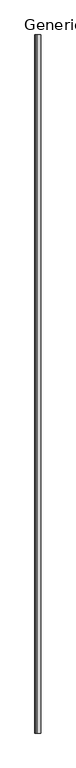
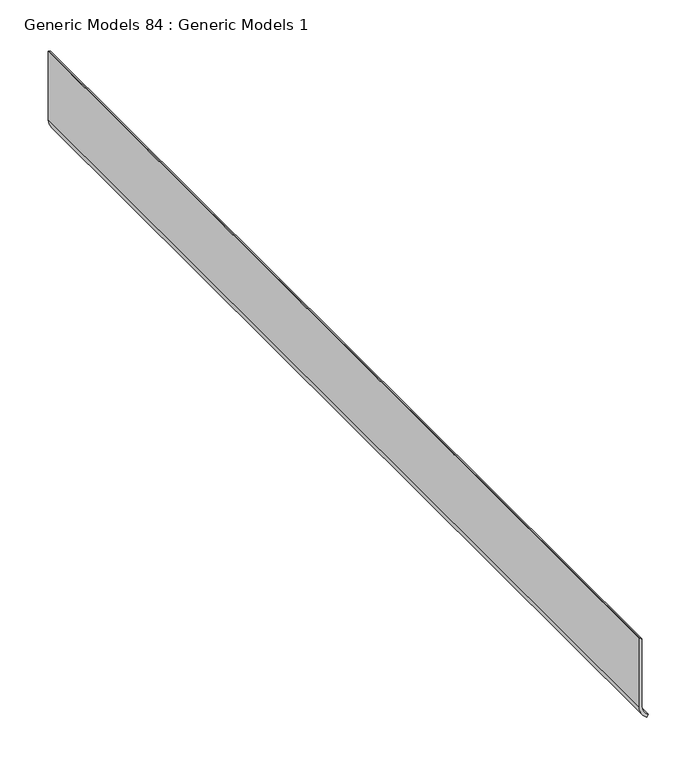
"""IFC4 building model written with IfcOpenShell, lengths in millimetres: proxy geometry, Generic Models 84 : Generic Models 1."""

from ifc_helpers import new_model, si_unit, point, frame, frame_2d, origin, place, context, project, spatial, polyline, circle_curve, trimmed, segment, composite_curve, outline, extrude, source, transform, mapped, element, save


def generic_models_84_generic_models_1_3640655c(model_context):
    return source(origin(), model_context, "Body", "SweptSolid", [
        extrude(outline(composite_curve([segment(polyline([(-124.376067, 46951.7485531), (-210.5264363, 46951.7485531)]), True, "CONTINUOUS"), segment(trimmed(circle_curve(frame_2d((-210.5264363, 46969.5882499)), 17.8396968), [point((-210.5264363, 46951.7485531))], [point((-225.976067, 46960.6684015))], False, "CARTESIAN"), True, "CONTINUOUS"), segment(polyline([(-225.976067, 46960.6684015), (-223.2264363, 46962.2559015)]), True, "CONTINUOUS"), segment(trimmed(circle_curve(frame_2d((-210.5264363, 46969.5882499)), 14.6646968), [point((-223.2264363, 46962.2559015))], [point((-210.5264363, 46954.9235531))], True, "CARTESIAN"), True, "CONTINUOUS"), segment(polyline([(-210.5264363, 46954.9235531), (-126.4628688, 46954.9235531)]), True, "CONTINUOUS"), segment(trimmed(circle_curve(frame_2d((-126.4628688, 46952.8367513)), 2.0868018), [point((-126.4628688, 46954.9235531))], [point((-124.376067, 46952.8367513))], False, "CARTESIAN"), True, "CONTINUOUS"), segment(polyline([(-124.376067, 46952.8367513), (-124.376067, 46951.7485531)]), True, "CONTINUOUS")], self_intersect=False)), frame((0.0, 0.0, 0.0), z_axis=(0.0, 1.0, 0.0), x_axis=(0.0, 0.0, 1.0)), (0.0, 0.0, 1.0), 1219.2),
    ])


if __name__ == "__main__":
    model = new_model("IFC4")
    model_context = context("Model", 3, world=origin())
    ifc_project = project(units=[si_unit("LENGTHUNIT", "METRE", prefix="MILLI")], contexts=[model_context])
    site = spatial("IfcSite", under=ifc_project)
    building = spatial("IfcBuilding", under=site)
    placement = place(None, origin())
    generic_models_84_generic_models_1_shape = generic_models_84_generic_models_1_3640655c(model_context)
    element("IfcBuildingElementProxy", 1, Name="Generic Models 84 : Generic Models 1", ObjectType="Generic Models 84 : Generic Models 1", at=placement, inside=building, context=model_context, shape_type="MappedRepresentation", body=[
        mapped(generic_models_84_generic_models_1_shape, transform((0.0, 0.0, 0.0), x_axis=(1.0, 0.0, 0.0), y_axis=(0.0, 1.0, 0.0), z_axis=(0.0, 0.0, 1.0))),
    ])
    save(model, "model.ifc")

# Revit data of these elements
# Element 1 (IfcBuildingElementProxy, "Generic Models 84 : Generic Models 1")
#   Materials on its faces: "MATCH EXISTING BASE"
# Materials
#   "MATCH EXISTING BASE": class "Generic", colour RGB 120 120 120, transparency 0, Cost = 0
